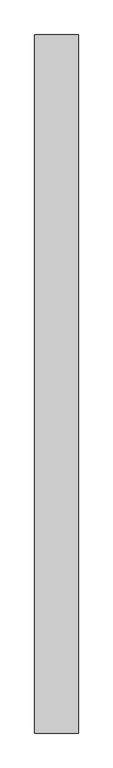
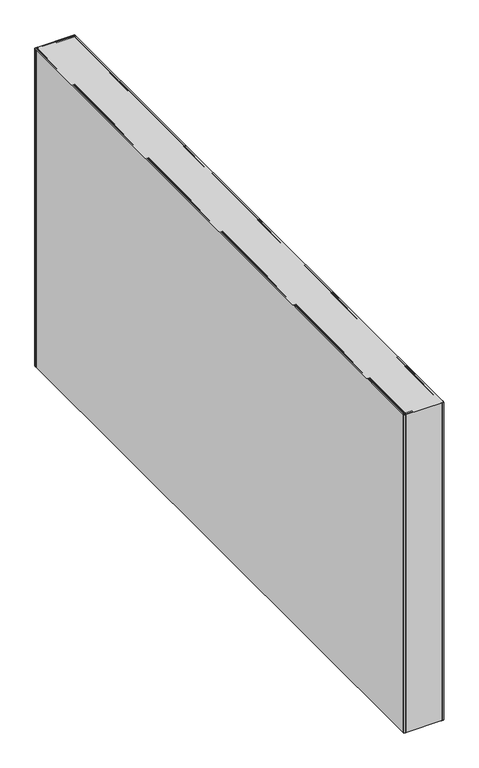
"""IFC4 building model written with IfcOpenShell, lengths in millimetres: beam geometry, LF02ZBK001_DIKE WALL_RC : Dike_Thk.250_EW3."""

from ifc_helpers import new_model, si_unit, origin, origin_with_axes, place, context, project, spatial, polyline, outline, extrude, source, transform, mapped, element, save


def beam_d64feadd(model_context):
    return source(origin(), model_context, "Body", "SweptSolid", [
        extrude(outline(polyline([(125.0, -2000.0), (-125.0, -2000.0), (-125.0, 2000.0), (125.0, 2000.0), (125.0, -2000.0)])), origin_with_axes(), (0.0, 0.0, 1.0), 2100.0),
        extrude(outline(polyline([(-125.0, -1985.0), (-125.0, -1984.0), (125.0, -1984.0), (125.0, -1985.0), (-125.0, -1985.0)])), origin_with_axes(), (0.0, 0.0, 1.0), 2100.0),
        extrude(outline(polyline([(-125.0, -1990.0), (-125.0, -1989.0), (125.0, -1989.0), (125.0, -1990.0), (-125.0, -1990.0)])), origin_with_axes(), (0.0, 0.0, 1.0), 2100.0),
        extrude(outline(polyline([(-125.0, -1995.0), (-125.0, -1994.0), (125.0, -1994.0), (125.0, -1995.0), (-125.0, -1995.0)])), origin_with_axes(), (0.0, 0.0, 1.0), 2100.0),
        extrude(outline(polyline([(-125.0, 1985.0), (125.0, 1985.0), (125.0, 1984.0), (-125.0, 1984.0), (-125.0, 1985.0)])), origin_with_axes(), (0.0, 0.0, 1.0), 2100.0),
        extrude(outline(polyline([(-125.0, 1990.0), (125.0, 1990.0), (125.0, 1989.0), (-125.0, 1989.0), (-125.0, 1990.0)])), origin_with_axes(), (0.0, 0.0, 1.0), 2100.0),
        extrude(outline(polyline([(-125.0, 1995.0), (125.0, 1995.0), (125.0, 1994.0), (-125.0, 1994.0), (-125.0, 1995.0)])), origin_with_axes(), (0.0, 0.0, 1.0), 2100.0),
        extrude(outline(polyline([(109.0, 2000.0), (110.0, 2000.0), (110.0, -2000.0), (109.0, -2000.0), (109.0, 2000.0)])), origin_with_axes(), (0.0, 0.0, 1.0), 2100.0),
        extrude(outline(polyline([(114.0, 2000.0), (115.0, 2000.0), (115.0, -2000.0), (114.0, -2000.0), (114.0, 2000.0)])), origin_with_axes(), (0.0, 0.0, 1.0), 2100.0),
        extrude(outline(polyline([(119.0, 2000.0), (120.0, 2000.0), (120.0, -2000.0), (119.0, -2000.0), (119.0, 2000.0)])), origin_with_axes(), (0.0, 0.0, 1.0), 2100.0),
        extrude(outline(polyline([(-109.0, 2000.0), (-109.0, -2000.0), (-110.0, -2000.0), (-110.0, 2000.0), (-109.0, 2000.0)])), origin_with_axes(), (0.0, 0.0, 1.0), 2100.0),
        extrude(outline(polyline([(-114.0, 2000.0), (-114.0, -2000.0), (-115.0, -2000.0), (-115.0, 2000.0), (-114.0, 2000.0)])), origin_with_axes(), (0.0, 0.0, 1.0), 2100.0),
        extrude(outline(polyline([(-119.0, 2000.0), (-119.0, -2000.0), (-120.0, -2000.0), (-120.0, 2000.0), (-119.0, 2000.0)])), origin_with_axes(), (0.0, 0.0, 1.0), 2100.0),
    ])


if __name__ == "__main__":
    model = new_model("IFC4")
    model_context = context("Model", 3, world=origin())
    ifc_project = project(units=[si_unit("LENGTHUNIT", "METRE", prefix="MILLI")], contexts=[model_context])
    site = spatial("IfcSite", under=ifc_project)
    building = spatial("IfcBuilding", under=site)
    placement = place(None, origin())
    beam_shape = beam_d64feadd(model_context)
    element("IfcBeam", 1, ObjectType="LF02ZBK001_DIKE WALL_RC : Dike_Thk.250_EW3", at=placement, inside=building, context=model_context, shape_type="MappedRepresentation", body=[
        mapped(beam_shape, transform((0.0, 0.0, 0.0), x_axis=(1.0, 0.0, 0.0), y_axis=(0.0, 1.0, 0.0), z_axis=(0.0, 0.0, 1.0))),
    ])
    save(model, "model.ifc")

# Revit data of these elements
# Type "LF02ZBK001_DIKE WALL_RC : Dike_Thk.250_EW3"
#   Dike_thk = 250 mm
#   Dike_Length [instance default] = 3000 mm
#   Dike_Hight = 2100 mm
#   c2_visible = yes
#   c3_material [instance default] = none
#   c2_material 3 [instance default] = none
#   c2_material 2 [instance default] = none
#   c2_material 1 [instance default] = none
#   c1_material [instance default] = none
#   Default Elevation = 0
# Element 1 (IfcBeam, "LF02ZBK001_DIKE WALL_RC : Dike_Thk.250_EW3")
#   Dike_Length = 4000 mm
